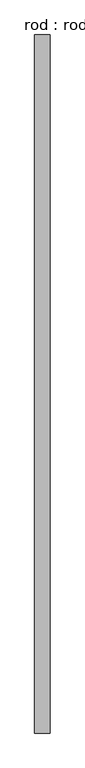
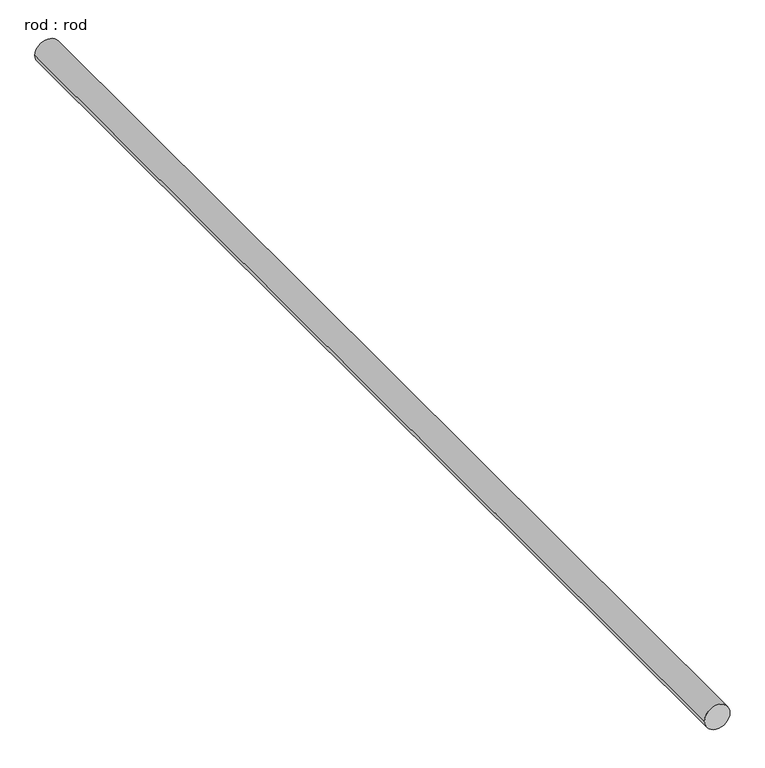
"""IFC4 building model written with IfcOpenShell, lengths in millimetres: proxy geometry, rod : rod."""

import ifcopenshell
import ifcopenshell.guid

model = None  # the IFC model being written
_history = None  # IfcOwnerHistory: only IFC2X3 demands one
_inside = {}  # id of a spatial element -> (the spatial element, [elements in it])
_under = {}  # id of a project, library or spatial element -> (it, [spatial elements below it])
_declared = {}  # id of a project -> (the project, [libraries it declares])
_typed = {}  # id of a type object -> (the type object, [elements of that type])
_made_of = {}  # id of a material, layer set ... -> (it, [elements and type objects made of it])


def new_model(schema):
    """Start an empty IFC model of exactly this schema.

    Asked for "IFC4X3", IfcOpenShell would pick the latest addendum, in which some entities
    have other attributes; the version numbers below select the first issue.
    IFC2X3 requires an IfcOwnerHistory on every rooted entity: one is made here for all.
    """
    global model, _history
    if schema == "IFC4X3":
        model = ifcopenshell.file(schema_version=(4, 3, 0, 0))
    else:
        model = ifcopenshell.file(schema=schema)
    _inside.clear()
    _under.clear()
    _declared.clear()
    _typed.clear()
    _made_of.clear()
    _history = None
    if model.schema == "IFC2X3":
        org = make("IfcOrganization", Name="unknown")
        user = make(
            "IfcPersonAndOrganization",
            ThePerson=make("IfcPerson", FamilyName="unknown"),
            TheOrganization=org,
        )
        app = make(
            "IfcApplication",
            ApplicationDeveloper=org,
            Version="unknown",
            ApplicationFullName="unknown",
            ApplicationIdentifier="unknown",
        )
        _history = make(
            "IfcOwnerHistory",
            OwningUser=user,
            OwningApplication=app,
            ChangeAction="ADDED",
            CreationDate=0,
        )
    return model


def make(cls, **values):
    """One entity of the class cls with the attributes given. An attribute that is None is left unset."""
    return model.create_entity(
        cls, **{name: value for name, value in values.items() if value is not None}
    )


def rooted(cls, **values):
    """An entity with a GlobalId (a new one), such as an element, a storey or a relation."""
    return make(cls, GlobalId=ifcopenshell.guid.new(), OwnerHistory=_history, **values)


def si_unit(unit_type, name, prefix=None):
    """IfcSIUnit, for example si_unit("LENGTHUNIT", "METRE", prefix="MILLI")."""
    return make("IfcSIUnit", UnitType=unit_type, Prefix=prefix, Name=name)


def assignment(units):
    """IfcUnitAssignment: the units of a project."""
    return None if units is None else make("IfcUnitAssignment", Units=units)


def point(xyz):
    """IfcCartesianPoint."""
    return None if xyz is None else make("IfcCartesianPoint", Coordinates=xyz)


def direction(xyz):
    """IfcDirection."""
    return None if xyz is None else make("IfcDirection", DirectionRatios=xyz)


def frame(location, z_axis=None, x_axis=None):
    """IfcAxis2Placement3D, a coordinate frame: its origin and axes. An axis left out is left unset."""
    return make(
        "IfcAxis2Placement3D",
        Location=point(location),
        Axis=direction(z_axis),
        RefDirection=direction(x_axis),
    )


def frame_2d(location, x_axis=None):
    """IfcAxis2Placement2D, a coordinate frame in the plane: its origin and x axis."""
    return make(
        "IfcAxis2Placement2D", Location=point(location), RefDirection=direction(x_axis)
    )


def origin():
    """The frame at (0, 0, 0) with its axes left unset."""
    return frame((0.0, 0.0, 0.0))


def place(relative_to, where):
    """IfcLocalPlacement: puts the frame where relative to a parent placement (None: the world)."""
    return make(
        "IfcLocalPlacement", PlacementRelTo=relative_to, RelativePlacement=where
    )


def context(
    kind, dimensions, precision=None, world=None, true_north=None, identifier=None
):
    """IfcGeometricRepresentationContext, for example the 3D "Model" context."""
    return make(
        "IfcGeometricRepresentationContext",
        ContextIdentifier=identifier,
        ContextType=kind,
        CoordinateSpaceDimension=dimensions,
        Precision=precision,
        WorldCoordinateSystem=world,
        TrueNorth=true_north,
    )


def project(units=None, contexts=None):
    """IfcProject with its units and contexts."""
    return rooted(
        "IfcProject",
        Name="project",
        RepresentationContexts=contexts,
        UnitsInContext=assignment(units),
    )


def spatial(cls, under=None, at=None, **own):
    """A site, building, storey or space (cls), placed at a placement, below another one or the project."""
    s = rooted(cls, ObjectPlacement=at, **own)
    if under is not None:
        _under.setdefault(under.id(), (under, []))[1].append(s)
    return s


def circle_curve(where, radius):
    """IfcCircle in the frame where."""
    return make("IfcCircle", Position=where, Radius=radius)


def trimmed(basis, trim1, trim2, sense, master):
    """IfcTrimmedCurve: the piece of a basis curve between two trims."""
    return make(
        "IfcTrimmedCurve",
        BasisCurve=basis,
        Trim1=trim1,
        Trim2=trim2,
        SenseAgreement=sense,
        MasterRepresentation=master,
    )


def segment(curve, same_sense, transition):
    """IfcCompositeCurveSegment."""
    return make(
        "IfcCompositeCurveSegment",
        Transition=transition,
        SameSense=same_sense,
        ParentCurve=curve,
    )


def composite_curve(segments, self_intersect=None):
    """IfcCompositeCurve: segments joined end to end."""
    return make("IfcCompositeCurve", Segments=segments, SelfIntersect=self_intersect)


def outline(outer, holes=None, kind="AREA"):
    """IfcArbitraryClosedProfileDef: a profile drawn as a closed curve; with holes, ...WithVoids."""
    if holes is None:
        return make("IfcArbitraryClosedProfileDef", ProfileType=kind, OuterCurve=outer)
    return make(
        "IfcArbitraryProfileDefWithVoids",
        ProfileType=kind,
        OuterCurve=outer,
        InnerCurves=holes,
    )


def extrude(swept, where, along, depth):
    """IfcExtrudedAreaSolid: the profile swept, set in the frame where, extruded along a direction by depth."""
    return make(
        "IfcExtrudedAreaSolid",
        SweptArea=swept,
        Position=where,
        ExtrudedDirection=direction(along),
        Depth=depth,
    )


def shape(context_of_items, identifier, shape_type, items):
    """IfcShapeRepresentation: the items that make up one representation, for example the "Body"."""
    return make(
        "IfcShapeRepresentation",
        ContextOfItems=context_of_items,
        RepresentationIdentifier=identifier,
        RepresentationType=shape_type,
        Items=items,
    )


def source(mapping_origin, context_of_items, identifier, shape_type, items):
    """IfcRepresentationMap: a shape defined once, which mapped items show again and again."""
    return make(
        "IfcRepresentationMap",
        MappingOrigin=mapping_origin,
        MappedRepresentation=shape(context_of_items, identifier, shape_type, items),
    )


def transform(
    local_origin,
    x_axis=None,
    y_axis=None,
    z_axis=None,
    scale=None,
    scale2=None,
    scale3=None,
    uniform=True,
):
    """IfcCartesianTransformationOperator3D, or its non-uniform kind. x_axis, y_axis, z_axis: its Axis1, 2, 3."""
    if uniform:
        return make(
            "IfcCartesianTransformationOperator3D",
            Axis1=direction(x_axis),
            Axis2=direction(y_axis),
            LocalOrigin=point(local_origin),
            Scale=scale,
            Axis3=direction(z_axis),
        )
    return make(
        "IfcCartesianTransformationOperator3DnonUniform",
        Axis1=direction(x_axis),
        Axis2=direction(y_axis),
        LocalOrigin=point(local_origin),
        Scale=scale,
        Axis3=direction(z_axis),
        Scale2=scale2,
        Scale3=scale3,
    )


def mapped(mapping_source, mapping_target):
    """IfcMappedItem: shows the shape of a source again, moved by a transform."""
    return make(
        "IfcMappedItem", MappingSource=mapping_source, MappingTarget=mapping_target
    )


def made_of(thing, what):
    """Note that an element or type object is made of a material, layer set ...; save() writes the relation."""
    if what is not None:
        _made_of.setdefault(what.id(), (what, []))[1].append(thing)
    return thing


def element(
    cls,
    number,
    at=None,
    inside=None,
    cuts=None,
    type_object=None,
    material=None,
    context=None,
    identifier="Body",
    shape_type=None,
    held_by="IfcProductDefinitionShape",
    body=None,
    shapes=None,
    **own,
):
    """One element of the class cls, such as IfcWall. Its Tag is "e" and its number.

    at: its placement. inside: the storey or other place that contains it. cuts: it is an
    opening in that element (IfcRelVoidsElement). A single representation is given by context,
    identifier, shape_type and body (its items); several are given by shapes. held_by: the class
    of the entity that holds the representations. save() writes the other relations.
    """
    e = rooted(cls, Tag="e%d" % number, ObjectPlacement=at, **own)
    if body is not None:
        shapes = [shape(context, identifier, shape_type, body)]
    if shapes is not None:
        e.Representation = make(held_by, Representations=shapes)
    if inside is not None:
        _inside.setdefault(inside.id(), (inside, []))[1].append(e)
    if cuts is not None:
        rooted(
            "IfcRelVoidsElement", RelatingBuildingElement=cuts, RelatedOpeningElement=e
        )
    if type_object is not None:
        _typed.setdefault(type_object.id(), (type_object, []))[1].append(e)
    return made_of(e, material)


def aggregate(whole, parts):
    """IfcRelAggregates: a whole, such as a stair, and the parts it consists of."""
    return rooted("IfcRelAggregates", RelatingObject=whole, RelatedObjects=parts)


def save(model, path):
    """Write the relations noted so far, then the file.

    IfcRelAggregates (storeys below a building ...), IfcRelContainedInSpatialStructure (elements
    in a storey), IfcRelDefinesByType, IfcRelAssociatesMaterial and IfcRelDeclares: one each for
    every whole, place, type object, material and project.
    """
    for whole, parts in _under.values():
        aggregate(whole, parts)
    for where, things in _inside.values():
        rooted(
            "IfcRelContainedInSpatialStructure",
            RelatedElements=things,
            RelatingStructure=where,
        )
    for kind, things in _typed.values():
        rooted("IfcRelDefinesByType", RelatedObjects=things, RelatingType=kind)
    for what, things in _made_of.values():
        rooted("IfcRelAssociatesMaterial", RelatedObjects=things, RelatingMaterial=what)
    for by, libraries in _declared.values():
        rooted("IfcRelDeclares", RelatingContext=by, RelatedDefinitions=libraries)
    model.write(path)


def rod_rod_e89f44aa(model_context):
    return source(origin(), model_context, "Body", "SweptSolid", [
        extrude(outline(composite_curve([segment(trimmed(circle_curve(frame_2d((0.0108462, 0.0)), 200.0), [point((0.0108462, 200.0))], [point((0.0108462, -200.0))], False, "CARTESIAN"), True, "CONTINUOUS"), segment(trimmed(circle_curve(frame_2d((0.0108462, 0.0)), 200.0), [point((0.0108462, -200.0))], [point((0.0108462, 200.0))], False, "CARTESIAN"), True, "CONTINUOUS")], self_intersect=False)), frame((0.0, -5032.2713847, 0.0), z_axis=(0.0, 1.0, 0.0), x_axis=(0.0, 0.0, 1.0)), (0.0, 0.0, 1.0), 18250.0),
    ])


if __name__ == "__main__":
    model = new_model("IFC4")
    model_context = context("Model", 3, world=origin())
    ifc_project = project(units=[si_unit("LENGTHUNIT", "METRE", prefix="MILLI")], contexts=[model_context])
    site = spatial("IfcSite", under=ifc_project)
    building = spatial("IfcBuilding", under=site)
    placement = place(None, origin())
    rod_rod_shape = rod_rod_e89f44aa(model_context)
    element("IfcBuildingElementProxy", 1, Name="rod : rod", ObjectType="rod : rod", at=placement, inside=building, context=model_context, shape_type="MappedRepresentation", body=[
        mapped(rod_rod_shape, transform((0.0, 0.0, 0.0), x_axis=(1.0, 0.0, 0.0), y_axis=(0.0, 1.0, 0.0), z_axis=(0.0, 0.0, 1.0))),
    ])
    save(model, "model.ifc")

# Revit data of these elements
# Type "rod : rod"
#   Default Elevation = 0
